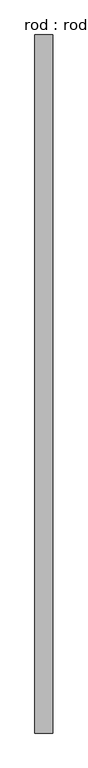
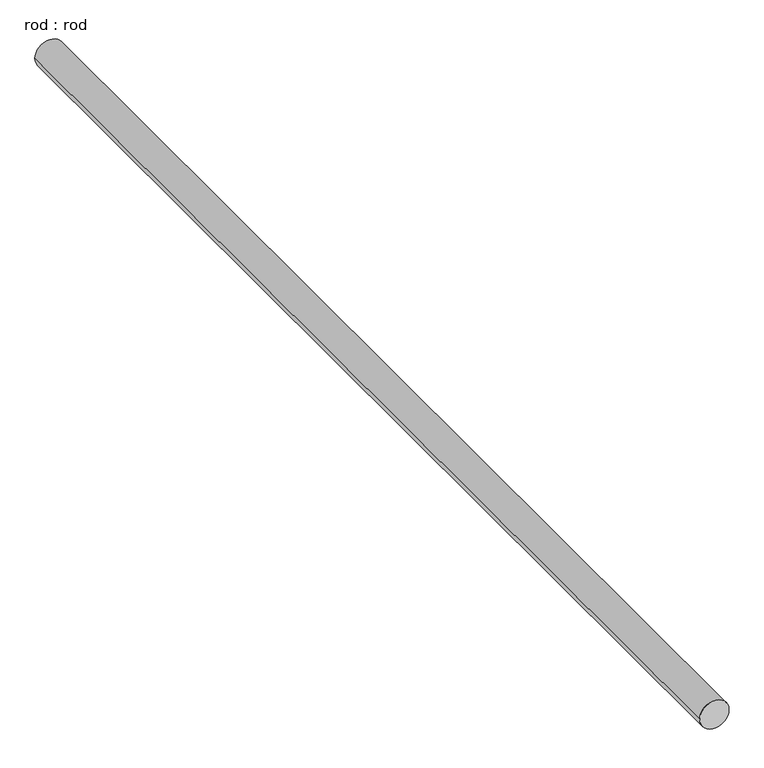
"""IFC4 building model written with IfcOpenShell, lengths in millimetres: proxy geometry, rod : rod."""

from ifc_helpers import new_model, si_unit, point, frame, frame_2d, origin, place, context, project, spatial, circle_curve, trimmed, segment, composite_curve, outline, extrude, source, transform, mapped, element, save


def rod_rod_7500283d(model_context):
    return source(origin(), model_context, "Body", "SweptSolid", [
        extrude(outline(composite_curve([segment(trimmed(circle_curve(frame_2d((0.0108462, 0.0)), 200.0), [point((0.0108462, 200.0))], [point((0.0108462, -200.0))], False, "CARTESIAN"), True, "CONTINUOUS"), segment(trimmed(circle_curve(frame_2d((0.0108462, 0.0)), 200.0), [point((0.0108462, -200.0))], [point((0.0108462, 200.0))], False, "CARTESIAN"), True, "CONTINUOUS")], self_intersect=False)), frame((0.0, -3801.0832411, 0.0), z_axis=(0.0, 1.0, 0.0), x_axis=(0.0, 0.0, 1.0)), (0.0, 0.0, 1.0), 15787.6237129),
    ])


if __name__ == "__main__":
    model = new_model("IFC4")
    model_context = context("Model", 3, world=origin())
    ifc_project = project(units=[si_unit("LENGTHUNIT", "METRE", prefix="MILLI")], contexts=[model_context])
    site = spatial("IfcSite", under=ifc_project)
    building = spatial("IfcBuilding", under=site)
    placement = place(None, origin())
    rod_rod_shape = rod_rod_7500283d(model_context)
    element("IfcBuildingElementProxy", 1, Name="rod : rod", ObjectType="rod : rod", at=placement, inside=building, context=model_context, shape_type="MappedRepresentation", body=[
        mapped(rod_rod_shape, transform((0.0, 0.0, 0.0), x_axis=(1.0, 0.0, 0.0), y_axis=(0.0, 1.0, 0.0), z_axis=(0.0, 0.0, 1.0))),
    ])
    save(model, "model.ifc")

# Revit data of these elements
# Type "rod : rod"
#   Default Elevation = 0
